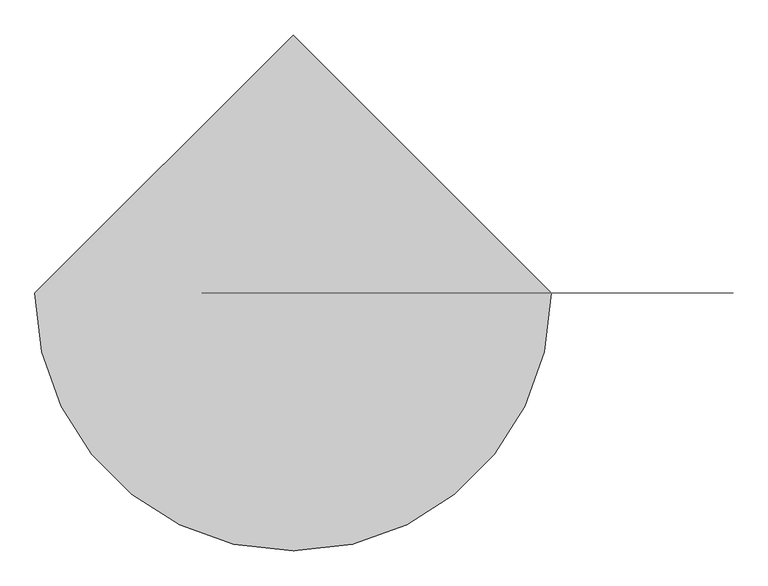
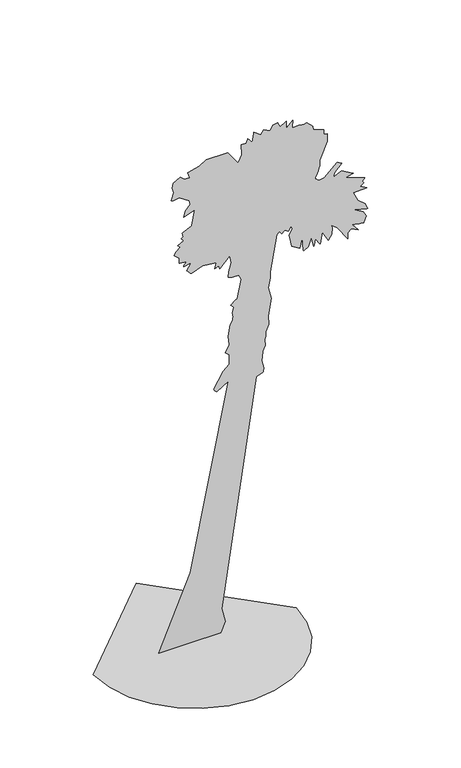
"""IFC4 building model written with IfcOpenShell, lengths in millimetres: proxy geometry, california fan palm 26448 : california fan palm 26448."""

from ifc_helpers import new_model, si_unit, origin, place, context, project, spatial, triangles, source, transform, mapped, element, save


def entourage_5d10e8ee(model_context):
    return source(origin(), model_context, "Body", "Tessellation", [
        triangles([(-2230.6788128, 0.0, 0.0), (-2171.7626415, -511.0878808, 0.0), (-2003.8055969, -980.4489481, 0.0), (-1740.3231331, -1394.6991714, 0.0), (-1394.6991714, -1740.3231331, 0.0), (-980.4489481, -2003.8055969, 0.0), (-511.0878808, -2171.7626415, 0.0), (0.0, -2230.6788128, 0.0), (511.0878808, -2171.7626415, 0.0), (980.4489481, -2003.8055969, 0.0), (1394.6991714, -1740.3231331, 0.0), (1740.3231331, -1394.6991714, 0.0), (2003.8055969, -980.4489481, 0.0), (2171.7626415, -511.0878808, 0.0), (2230.6788128, 0.0, 0.0), (0.0, 2230.6788128, 0.0), (1664.2176041, 0.0, 11296.8139435), (1716.9665646, 0.0, 11409.2663818), (1822.5957275, 0.0, 11429.86745), (1831.5184387, 0.0, 11420.4191895), (1867.2094288, 0.0, 11334.210498), (1869.9649292, 0.0, 11312.4281067), (2015.4839539, 0.0, 11398.3751862), (2017.4521477, 0.0, 11231.8609314), (2029.3928432, 0.0, 11239.7348694), (2152.211364, 0.0, 11376.1997955), (2149.9806862, 0.0, 11207.8484436), (2152.473848, 0.0, 11197.3514099), (2288.0203709, 0.0, 11209.0297668), (2303.3726315, 0.0, 11206.5368958), (2322.5303284, 0.0, 11201.6813782), (2343.1312511, 0.0, 11196.0398621), (2362.6825287, 0.0, 11190.7901825), (2378.8220959, 0.0, 11187.6415375), (2392.5998886, 0.0, 11190.1344086), (2470.1486435, 0.0, 11209.9483154), (2596.1165359, 0.0, 11074.5333252), (2606.0888924, 0.0, 10999.6088287), (2622.0972176, 0.0, 10989.2420197), (2841.8846741, 0.0, 10912.2188141), (2834.4054794, 0.0, 10804.8835052), (2918.2526871, 0.0, 10792.4179871), (2914.3162994, 0.0, 10622.229538), (2746.3591095, 0.0, 10233.4358276), (2746.8840775, 0.0, 10223.5945679), (2748.4586906, 0.0, 10207.4548553), (2750.2957878, 0.0, 10187.6409485), (2752.0014977, 0.0, 10166.9096558), (2753.1825302, 0.0, 10147.8829102), (2752.5264656, 0.0, 10129.2503265), (2746.4904968, 0.0, 10101.3008698), (2732.5814621, 0.0, 10059.0487976), (2713.4239105, 0.0, 10006.1694672), (2692.2981651, 0.0, 9950.4019409), (2672.3531616, 0.0, 9899.7527069), (2657.000901, 0.0, 9861.830603), (2649.652803, 0.0, 9844.3793427), (2655.1638039, 0.0, 9835.7194061), (2666.9732574, 0.0, 9823.9096619), (2682.588002, 0.0, 9810.3942078), (2699.9087471, 0.0, 9796.4857544), (2716.8356209, 0.0, 9783.8888489), (2731.1382362, 0.0, 9773.7848145), (2743.9973351, 0.0, 9768.1421356), (2762.8924026, 0.0, 9771.5535553), (2783.4934708, 0.0, 9776.0149109), (2805.8002487, 0.0, 9781.0018158), (2826.6638008, 0.0, 9785.987558), (2846.6085136, 0.0, 9790.8430756), (3136.3344337, 0.0, 10050.2574738), (3236.3213539, 0.0, 9997.9025299), (3081.0921661, 0.0, 9835.4566315), (3047.3698059, 0.0, 9739.0125183), (3230.9414497, 0.0, 9821.1540161), (3471.198587, 0.0, 9683.1141861), (3486.2886543, 0.0, 9668.9429581), (3314.6575607, 0.0, 9631.5464035), (3745.0472786, 0.0, 9483.4031204), (3683.7693329, 0.0, 9424.0927872), (3714.4738541, 0.0, 9372.0000366), (3638.7619057, 0.0, 9318.7265442), (3786.6429955, 0.0, 9226.0874313), (3491.0122032, 0.0, 9221.3638824), (3589.5558975, 0.0, 9011.2860077), (3750.2957954, 0.0, 8872.4595978), (3802.1263527, 0.0, 8753.0523514), (3802.3888367, 0.0, 8743.6046722), (3785.8555435, 0.0, 8741.1118011), (3521.0609505, 0.0, 8817.3484268), (3708.9628532, 0.0, 8702.927504), (3773.3900253, 0.0, 8589.950679), (3773.3900253, 0.0, 8579.0594833), (3723.3965652, 0.0, 8451.5172684), (3722.7405006, 0.0, 8439.9702988), (3582.3388962, 0.0, 8467.3942062), (3469.6239738, 0.0, 8483.9274994), (3593.2298012, 0.0, 8317.5452133), (3446.0050667, 0.0, 8391.1575806), (3364.6510208, 0.0, 8326.0743439), (3364.9135048, 0.0, 8189.871611), (3139.2211761, 0.0, 8528.6724426), (3001.4438301, 0.0, 8636.6635254), (3024.9316406, 0.0, 8566.4625778), (3019.5517365, 0.0, 8420.4185852), (2940.4283684, 0.0, 8304.6861145), (2805.2752808, 0.0, 8540.6129929), (2760.1370476, 0.0, 8283.0351105), (2749.7708199, 0.0, 8292.6141769), (2653.9827713, 0.0, 8439.0517502), (2626.9524445, 0.0, 8297.7313065), (2620.9164757, 0.0, 8283.0351105), (2579.5832428, 0.0, 8449.8115585), (2567.9048859, 0.0, 8491.0131134), (2498.0978096, 0.0, 8313.2152451), (2400.9976318, 0.0, 8247.8692337), (2391.943824, 0.0, 8267.9453339), (2363.6010773, 0.0, 8580.3716125), (2316.2318756, 0.0, 8342.0826691), (2134.3659416, 0.0, 8446.7931381), (2079.2550613, 0.0, 8724.578508), (2142.2390076, 0.0, 8848.577916), (2140.5331524, 0.0, 8863.4054993), (2136.7278614, 0.0, 8876.1332108), (2131.7416832, 0.0, 8889.1236969), (2126.493021, 0.0, 8901.1956345), (2118.2263744, 0.0, 8911.5618622), (2064.821204, 0.0, 8836.1123978), (2061.278397, 0.0, 8825.74617), (1984.5168034, 0.0, 8874.5588882), (1971.6575592, 0.0, 8870.8846939), (1961.5539608, 0.0, 8863.4054993), (1929.4059231, 0.0, 8825.3525894), (1918.6462601, 0.0, 8820.3662659), (1866.2908802, 0.0, 8885.1873093), (1856.7121044, 0.0, 8882.4316635), (1845.5587154, 0.0, 8875.3460495), (1833.7492619, 0.0, 8865.5047897), (1822.2021469, 0.0, 8854.2200134), (1811.8360645, 0.0, 8842.9358185), (1800.8139175, 0.0, 8829.6825577), (1660.4123131, 0.0, 8018.3716141), (1661.7244423, 0.0, 7883.0874298), (1618.029435, 0.0, 7666.7116837), (1684.0312202, 0.0, 7392.9946701), (1613.6993214, 0.0, 6996.1962158), (1630.1013725, 0.0, 6826.0083481), (1628.2642754, 0.0, 6813.1492493), (1565.0179905, 0.0, 6658.9697067), (1565.0179905, 0.0, 6648.2098984), (1564.7555065, 0.0, 6634.432251), (1564.2306839, 0.0, 6619.0802811), (1564.0994419, 0.0, 6603.3341492), (1564.3619259, 0.0, 6588.6379532), (1566.3301197, 0.0, 6572.10466), (1566.0677811, 0.0, 6561.3448517), (1562.0000061, 0.0, 6547.1736237), (1555.9640373, 0.0, 6528.54104), (1549.2720039, 0.0, 6508.2021652), (1542.9736965, 0.0, 6489.176001), (1536.6752438, 0.0, 6470.41203), (1549.6657299, 0.0, 6358.8781403), (1547.8286327, 0.0, 6349.0368805), (1519.879612, 0.0, 6273.9809967), (1509.1198036, 0.0, 6246.9500885), (1500.7219151, 0.0, 6225.4310532), (1496.3918015, 0.0, 6213.6213089), (1479.0712017, 0.0, 6016.271727), (1517.6489342, 0.0, 5834.537471), (1516.3366596, 0.0, 5819.7098877), (1513.5811592, 0.0, 5801.6016907), (1510.1695942, 0.0, 5782.7069138), (1506.6266418, 0.0, 5765.255072), (1502.4277702, 0.0, 5747.9346176), (1492.9802364, 0.0, 5740.5862289), (1349.2983089, 0.0, 5680.8828964), (595.4600201, 0.0, 547.8284798), (673.9273962, 0.0, 229.1038392), (568.9542978, 0.0, 0.0), (-790.1851255, 0.0, 0.0), (-95.6567521, 0.0, 1632.0695663), (739.9292542, 0.0, 5779.1641068), (737.436165, 0.0, 5791.104657), (723.0023804, 0.0, 5788.3490112), (497.4413664, 0.0, 5642.1742126), (481.6954162, 0.0, 5644.929277), (467.1303895, 0.0, 5652.2776657), (442.9865507, 0.0, 5676.2901535), (421.4670794, 0.0, 5718.8044189), (623.2778715, 0.0, 6073.2199951), (759.0868784, 0.0, 6187.6403366), (764.0731293, 0.0, 6248.393605), (761.5799675, 0.0, 6329.354361), (759.4805317, 0.0, 6365.176593), (758.0371605, 0.0, 6391.1569839), (755.0191761, 0.0, 6405.9845673), (666.1856449, 0.0, 6482.8775482), (763.548234, 0.0, 6634.301445), (735.9927938, 0.0, 6838.6052536), (766.6974604, 0.0, 7041.3347397), (776.8010588, 0.0, 7092.5089417), (840.0474163, 0.0, 7190.1337967), (839.522521, 0.0, 7202.4679276), (839.653763, 0.0, 7214.1462845), (840.3098276, 0.0, 7226.8745773), (841.2283762, 0.0, 7239.2087082), (843.0654007, 0.0, 7253.5113235), (843.459054, 0.0, 7264.4025192), (841.4907875, 0.0, 7278.1801666), (838.3415611, 0.0, 7296.025589), (834.5362701, 0.0, 7315.1831406), (830.9934631, 0.0, 7332.8971756), (827.1881721, 0.0, 7349.5618561), (858.9425566, 0.0, 7476.4482971), (792.0222227, 0.0, 7542.3186951), (801.9946518, 0.0, 7559.2455688), (893.5836834, 0.0, 7626.0345154), (936.6226988, 0.0, 7645.4548416), (1020.8635597, 0.0, 8067.9714935), (970.6076883, 0.0, 8186.4601913), (830.0749146, 0.0, 8178.4560287), (740.9790447, 0.0, 8214.1468735), (747.8022474, 0.0, 8345.4940887), (801.8634098, 0.0, 8532.8710236), (775.3576876, 0.0, 8707.5202469), (545.597802, 0.0, 8480.6468857), (527.0962787, 0.0, 8557.4084793), (442.0680385, 0.0, 8522.5053772), (472.772705, 0.0, 8646.6361725), (175.6987596, 0.0, 8679.0464035), (149.3242611, 0.0, 8677.3406937), (-68.4949607, 0.0, 8593.099324), (-83.7160656, 0.0, 8594.6742279), (-100.2493315, 0.0, 8606.0898102), (-163.6268583, 0.0, 8679.0464035), (-174.6490235, 0.0, 8687.0505661), (-73.2187503, 0.0, 8837.8181076), (-247.211691, 0.0, 8810.3942001), (-243.8000715, 0.0, 8822.3347504), (-191.1822985, 0.0, 8889.9108582), (-182.5220168, 0.0, 8896.9970535), (-226.4795081, 0.0, 8901.4584091), (-326.8600634, 0.0, 8910.7747009), (-336.4388391, 0.0, 8914.1861206), (-338.5383113, 0.0, 9032.0184631), (-454.139976, 0.0, 9130.9554474), (-421.729527, 0.0, 9200.631427), (-316.4939446, 0.0, 9287.7592484), (-374.0979504, 0.0, 9343.1326126), (-245.112237, 0.0, 9404.9352356), (-247.8677738, 0.0, 9414.1207214), (-255.0846843, 0.0, 9424.7491425), (-300.8792001, 0.0, 9470.2812469), (-254.166172, 0.0, 9507.1528336), (-275.2920083, 0.0, 9598.0862366), (-268.468751, 0.0, 9606.3525925), (-79.1234862, 0.0, 9686.3947998), (-65.8706341, 0.0, 9707.3894485), (-0.1312164, 0.0, 10040.1546021), (-244.7185837, 0.0, 9956.7003937), (-207.9780029, 0.0, 10078.3383179), (-100.1181167, 0.0, 10203.780661), (-126.0989619, 0.0, 10300.0933868), (-346.8049579, 0.0, 10440.889444), (-468.442555, 0.0, 10419.7628265), (-522.8973707, 0.0, 10436.8210876), (-465.9494296, 0.0, 10603.5969543), (-492.9800108, 0.0, 10720.6421356), (-468.8362083, 0.0, 10823.2533142), (-318.9870701, 0.0, 10910.9061035), (-233.6964004, 0.0, 10839.2616394), (-108.1223157, 0.0, 10825.353186), (-151.5549389, 0.0, 10960.7681763), (96.9689176, 0.0, 11018.8971863), (255.6095432, 0.0, 11124.9197845), (725.2330582, 0.0, 11114.0285889), (954.2056372, 0.0, 10789.530954), (960.8976706, 0.0, 10798.7164398), (1037.2656109, 0.0, 10964.7051453), (1025.8498106, 0.0, 11198.2699585), (1137.9085957, 0.0, 11192.758667), (1136.4652245, 0.0, 11204.0440247), (1141.5826447, 0.0, 11231.8609314), (1162.0524708, 0.0, 11273.5886169), (1170.1878754, 0.0, 11283.6914886), (1265.188472, 0.0, 11172.5517609), (1295.1058319, 0.0, 11376.1997955), (1299.9609135, 0.0, 11390.6337982), (1447.8417126, 0.0, 11287.365683), (1520.9292572, 0.0, 11379.6112152)], [[15, 16, 1], [14, 15, 1], [14, 1, 2], [13, 14, 2], [13, 2, 3], [13, 3, 4], [12, 13, 4], [11, 12, 4], [11, 4, 5], [11, 5, 6], [11, 6, 7], [11, 7, 8], [11, 8, 9], [11, 9, 10], [266, 267, 268], [266, 268, 269], [266, 269, 270], [271, 272, 273], [278, 279, 280], [283, 284, 285], [282, 283, 285], [281, 282, 285], [280, 281, 285], [278, 280, 285], [277, 278, 285], [286, 287, 288], [285, 286, 288], [277, 285, 288], [288, 289, 17], [277, 288, 17], [276, 277, 17], [18, 19, 20], [17, 18, 20], [17, 20, 21], [17, 21, 22], [22, 23, 24], [25, 26, 27], [25, 27, 28], [24, 25, 28], [35, 36, 37], [35, 37, 38], [34, 35, 38], [39, 40, 41], [41, 42, 43], [41, 43, 44], [39, 41, 44], [38, 39, 44], [34, 38, 44], [33, 34, 44], [32, 33, 44], [31, 32, 44], [30, 31, 44], [29, 30, 44], [28, 29, 44], [24, 28, 44], [70, 71, 72], [69, 70, 72], [69, 72, 73], [75, 76, 77], [74, 75, 77], [73, 74, 77], [77, 78, 79], [79, 80, 81], [77, 79, 81], [81, 82, 83], [77, 81, 83], [73, 77, 83], [86, 87, 88], [85, 86, 88], [84, 85, 88], [84, 88, 89], [83, 84, 89], [93, 94, 95], [92, 93, 95], [91, 92, 95], [90, 91, 95], [90, 95, 96], [96, 97, 98], [99, 100, 101], [98, 99, 101], [96, 98, 101], [90, 96, 101], [89, 90, 101], [89, 101, 102], [83, 89, 102], [73, 83, 102], [69, 73, 102], [68, 69, 102], [67, 68, 102], [66, 67, 102], [65, 66, 102], [64, 65, 102], [104, 105, 106], [103, 104, 106], [102, 103, 106], [64, 102, 106], [106, 107, 108], [106, 108, 109], [110, 111, 112], [109, 110, 112], [106, 109, 112], [106, 112, 113], [64, 106, 113], [114, 115, 116], [113, 114, 116], [113, 116, 117], [64, 113, 117], [117, 118, 119], [117, 119, 120], [117, 120, 121], [64, 117, 121], [64, 121, 122], [64, 122, 123], [64, 123, 124], [64, 124, 125], [64, 125, 126], [63, 64, 126], [62, 63, 126], [61, 62, 126], [60, 61, 126], [59, 60, 126], [58, 59, 126], [57, 58, 126], [127, 128, 129], [126, 127, 129], [57, 126, 129], [57, 129, 130], [131, 132, 133], [131, 133, 134], [130, 131, 134], [57, 130, 134], [177, 178, 179], [176, 177, 179], [176, 179, 180], [175, 176, 180], [175, 180, 181], [175, 181, 182], [187, 188, 189], [186, 187, 189], [185, 186, 189], [184, 185, 189], [183, 184, 189], [182, 183, 189], [182, 189, 190], [175, 182, 190], [175, 190, 191], [174, 175, 191], [173, 174, 191], [172, 173, 191], [171, 172, 191], [170, 171, 191], [169, 170, 191], [168, 169, 191], [167, 168, 191], [166, 167, 191], [166, 191, 192], [165, 166, 192], [165, 192, 193], [164, 165, 193], [164, 193, 194], [163, 164, 194], [163, 194, 195], [162, 163, 195], [161, 162, 195], [160, 161, 195], [159, 160, 195], [158, 159, 195], [157, 158, 195], [156, 157, 195], [155, 156, 195], [154, 155, 195], [153, 154, 195], [152, 153, 195], [151, 152, 195], [150, 151, 195], [149, 150, 195], [148, 149, 195], [148, 195, 196], [148, 196, 197], [148, 197, 198], [148, 198, 199], [147, 148, 199], [146, 147, 199], [145, 146, 199], [145, 199, 200], [145, 200, 201], [144, 145, 201], [144, 201, 202], [144, 202, 203], [144, 203, 204], [144, 204, 205], [144, 205, 206], [144, 206, 207], [143, 144, 207], [143, 207, 208], [143, 208, 209], [143, 209, 210], [143, 210, 211], [143, 211, 212], [143, 212, 213], [213, 214, 215], [213, 215, 216], [213, 216, 217], [143, 213, 217], [143, 217, 218], [142, 143, 218], [141, 142, 218], [141, 218, 219], [220, 221, 222], [220, 222, 223], [219, 220, 223], [141, 219, 223], [140, 141, 223], [140, 223, 224], [139, 140, 224], [138, 139, 224], [224, 225, 226], [226, 227, 228], [224, 226, 228], [234, 235, 236], [233, 234, 236], [232, 233, 236], [231, 232, 236], [230, 231, 236], [229, 230, 236], [236, 237, 238], [236, 238, 239], [236, 239, 240], [242, 243, 244], [241, 242, 244], [244, 245, 246], [244, 246, 247], [241, 244, 247], [240, 241, 247], [247, 248, 249], [240, 247, 249], [236, 240, 249], [229, 236, 249], [228, 229, 249], [224, 228, 249], [138, 224, 249], [137, 138, 249], [137, 249, 250], [136, 137, 250], [135, 136, 250], [135, 250, 251], [251, 252, 253], [135, 251, 253], [253, 254, 255], [253, 255, 256], [135, 253, 256], [135, 256, 257], [135, 257, 258], [134, 135, 258], [57, 134, 258], [56, 57, 258], [55, 56, 258], [54, 55, 258], [53, 54, 258], [52, 53, 258], [51, 52, 258], [50, 51, 258], [49, 50, 258], [48, 49, 258], [47, 48, 258], [46, 47, 258], [45, 46, 258], [44, 45, 258], [24, 44, 258], [22, 24, 258], [17, 22, 258], [276, 17, 258], [259, 260, 261], [258, 259, 261], [276, 258, 261], [276, 261, 262], [275, 276, 262], [274, 275, 262], [273, 274, 262], [271, 273, 262], [271, 262, 263], [270, 271, 263], [266, 270, 263], [266, 263, 264], [266, 264, 265]], closed=False),
    ])


if __name__ == "__main__":
    model = new_model("IFC4")
    model_context = context("Model", 3, world=origin())
    ifc_project = project(units=[si_unit("LENGTHUNIT", "METRE", prefix="MILLI")], contexts=[model_context])
    site = spatial("IfcSite", under=ifc_project)
    building = spatial("IfcBuilding", under=site)
    placement = place(None, origin())
    entourage_shape = entourage_5d10e8ee(model_context)
    element("IfcBuildingElementProxy", 1, Name="california fan palm 26448 : california fan palm 26448", ObjectType="california fan palm 26448 : california fan palm 26448", at=placement, inside=building, context=model_context, shape_type="MappedRepresentation", body=[
        mapped(entourage_shape, transform((0.0, 0.0, 0.0), x_axis=(1.0, 0.0, 0.0), y_axis=(0.0, 1.0, 0.0), z_axis=(0.0, 0.0, 1.0))),
    ])
    save(model, "model.ifc")

# Revit data of these elements
# Type "california fan palm 26448 : california fan palm 26448"
#   built-in parameter 1005195 = "RPC-16-1C97-WEA8-8LP7-XB2E-SRLV-LDXM-F4"
#   Height = 0
